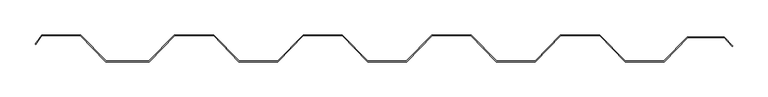
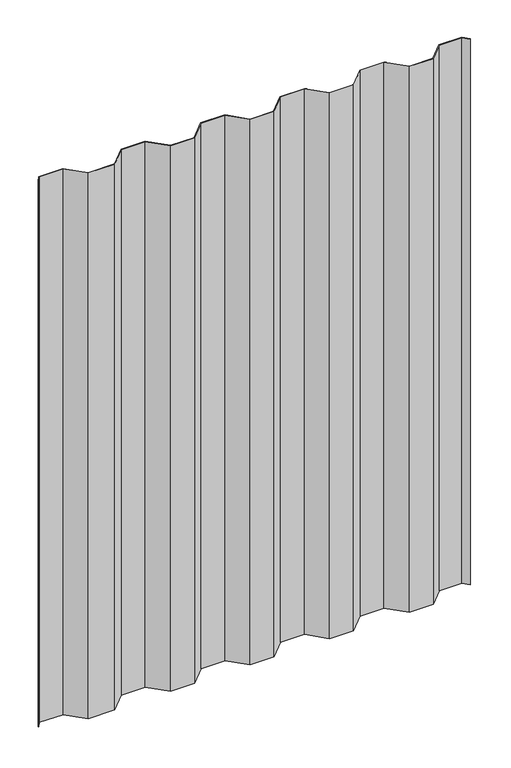
"""IFC4 building model written with IfcOpenShell, lengths in millimetres: proxy geometry, Generic Models 2:Generic Models 2:310765:Generic Models 2:310765 : Generic Models 2:Generic Models 2:310765:10 : Generic Models 2:Generic Models 2:310765:Generic Models 2:310765 : Generic Models 2:Generic Models 2:310765:300385."""

from ifc_helpers import new_model, si_unit, frame, origin, place, context, project, spatial, polyline, outline, extrude, source, transform, mapped, element, save


def generic_models_5e84f85a(model_context):
    return source(origin(), model_context, "Body", "SweptSolid", [
        extrude(outline(polyline([(579044.8590828, -578743.0895468), (579056.7148291, -578756.1976178), (579056.1528573, -578756.7595896), (579044.5067455, -578743.8832968), (578992.6003915, -578743.8832968), (578958.9684067, -578778.441384), (578903.7888468, -578778.441384), (578867.6266551, -578741.135134), (578812.2515295, -578741.135134), (578776.0893379, -578778.441384), (578720.9088468, -578778.441384), (578684.7466551, -578741.135134), (578629.3715295, -578741.135134), (578593.2093379, -578778.441384), (578538.0288468, -578778.441384), (578501.8666551, -578741.135134), (578446.4915295, -578741.135134), (578410.3293379, -578778.441384), (578355.1488468, -578778.441384), (578318.9866551, -578741.135134), (578263.6115295, -578741.135134), (578227.4493379, -578778.441384), (578165.9188468, -578778.441384), (578129.7566551, -578741.135134), (578075.2280924, -578741.135134), (578066.2867241, -578753.9047313), (578065.6365222, -578753.449455), (578074.8148923, -578740.341384), (578130.0927007, -578740.341384), (578166.2548923, -578777.647634), (578227.1132923, -578777.647634), (578263.275484, -578740.341384), (578319.3227007, -578740.341384), (578355.4848923, -578777.647634), (578409.9932923, -578777.647634), (578446.155484, -578740.341384), (578502.2027007, -578740.341384), (578538.3648923, -578777.647634), (578592.8732923, -578777.647634), (578629.035484, -578740.341384), (578685.0827007, -578740.341384), (578721.2448923, -578777.647634), (578775.7532923, -578777.647634), (578811.915484, -578740.341384), (578867.9627007, -578740.341384), (578904.1248923, -578777.647634), (578958.6332923, -578777.647634), (578992.2652771, -578743.0895468), (579044.8590828, -578743.0895468)])), frame((0.0, 0.0, 4828.849258), z_axis=(0.0, 0.0, 1.0), x_axis=(1.0, 0.0, 0.0)), (0.0, 0.0, 1.0), 1324.3203982),
    ])


if __name__ == "__main__":
    model = new_model("IFC4")
    model_context = context("Model", 3, world=origin())
    ifc_project = project(units=[si_unit("LENGTHUNIT", "METRE", prefix="MILLI")], contexts=[model_context])
    site = spatial("IfcSite", under=ifc_project)
    building = spatial("IfcBuilding", under=site)
    placement = place(None, origin())
    generic_models_shape = generic_models_5e84f85a(model_context)
    element("IfcBuildingElementProxy", 1, Name="Generic Models 2:Generic Models 2:310765:Generic Models 2:310765 : Generic Models 2:Generic Models 2:310765:10 : Generic Models 2:Generic Models 2:310765:Generic Models 2:310765 : Generic Models 2:Generic Models 2:310765:300385", ObjectType="Generic Models 2:Generic Models 2:310765:Generic Models 2:310765 : Generic Models 2:Generic Models 2:310765:10 : Generic Models 2:Generic Models 2:310765:Generic Models 2:310765 : Generic Models 2:Generic Models 2:310765:300385", at=placement, inside=building, context=model_context, shape_type="MappedRepresentation", body=[
        mapped(generic_models_shape, transform((0.0, 0.0, 0.0), x_axis=(1.0, 0.0, 0.0), y_axis=(0.0, 1.0, 0.0), z_axis=(0.0, 0.0, 1.0))),
    ])
    save(model, "model.ifc")

# Revit data of these elements
# Type "Generic Models 2:Generic Models 2:310765:Generic Models 2:310765 : Generic Models 2:Generic Models 2:310765:10 : Generic Models 2:Generic Models 2:310765:Generic Models 2:310765 : Generic Models 2:Generic Models 2:310765:300385"
#   NameOverride = "Generic Models 2:Generic Models 2:310765:Generic Models 2:310765 : Generic Models 2:Generic Models 2:310765:300385"
#   ObjectTypeOverride = "Generic Models 2:310765 : Generic Models 2:Generic Models 2:310765"
#   Reference = "Generic Models 2"
#   Tag = "300385"
# Element 1 (IfcBuildingElementProxy, "Generic Models 2:Generic Models 2:310765:Generic Models 2:310765 : Generic Models 2:Generic Models 2:310765:10 : Generic Models 2:Generic Models 2:310765:Generic Models 2:310765 : Generic Models 2:Generic Models 2:310765:300385")
#   Materials on its faces: "VERTICAL CORRUGATED METAL PANEL - EXPOSED FASTENERS - (MBCI 7.2 PANEL)"
# Materials
#   "VERTICAL CORRUGATED METAL PANEL - EXPOSED FASTENERS - (MBCI 7.2 PANEL)": class "Generic", colour RGB 120 120 120, transparency 0, Cost = 0
